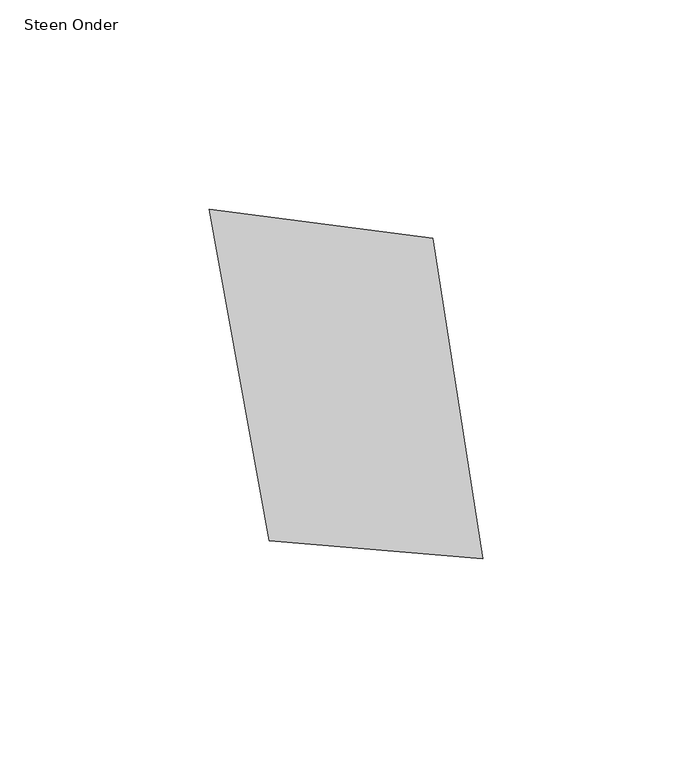
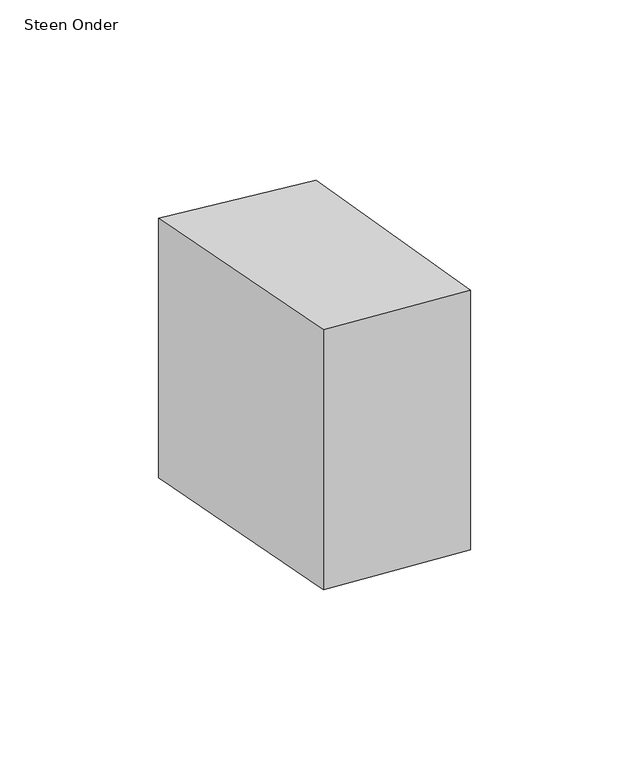
"""IFC4 building model written with IfcOpenShell, lengths in millimetres: proxy geometry, 00_GMA_steen_versie_4 : Steen Onder."""

from ifc_helpers import new_model, si_unit, origin, origin_with_axes, place, context, project, spatial, polyline, outline, extrude, source, transform, mapped, element, save


def steen_onder_d6d9aff7(model_context):
    return source(origin(), model_context, "Body", "SweptSolid", [
        extrude(outline(polyline([(94.9672766, 105.0774172), (106.9842773, 28.3403043), (55.8721666, 32.6517562), (41.5209664, 112.0147443), (94.9672766, 105.0774172)])), origin_with_axes(), (0.0, 0.0, 1.0), 100.0),
    ])


if __name__ == "__main__":
    model = new_model("IFC4")
    model_context = context("Model", 3, world=origin())
    ifc_project = project(units=[si_unit("LENGTHUNIT", "METRE", prefix="MILLI")], contexts=[model_context])
    site = spatial("IfcSite", under=ifc_project)
    building = spatial("IfcBuilding", under=site)
    placement = place(None, origin())
    steen_onder_shape = steen_onder_d6d9aff7(model_context)
    element("IfcBuildingElementProxy", 1, Name="00_GMA_steen_versie_4 : Steen Onder", ObjectType="00_GMA_steen_versie_4 : Steen Onder", at=placement, inside=building, context=model_context, shape_type="MappedRepresentation", body=[
        mapped(steen_onder_shape, transform((0.0, 0.0, 0.0), x_axis=(1.0, 0.0, 0.0), y_axis=(0.0, 1.0, 0.0), z_axis=(0.0, 0.0, 1.0))),
    ])
    save(model, "model.ifc")

# Revit data of these elements
# Type "00_GMA_steen_versie_4 : Steen Onder"
#   StootVoegHalfBoven [instance default] = 5 mm
#   StootVoegHalf [instance default] = 5 mm
#   StootVoegBreedteOnder = 10 mm
#   StootVoegBreedteBoven = 10 mm
#   Steendikte = 100 mm
#   LintVoegOnderHalf = 0 mm
#   LintVoegOnder = 0 mm
#   LintVoegBovenHalf = 5 mm
#   LintVoegBoven = 10 mm
#   materiaal = none
#   MateriaalVoeg = none
#   Default Elevation = 0
